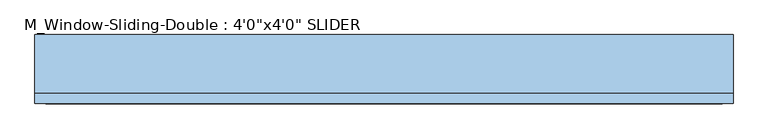
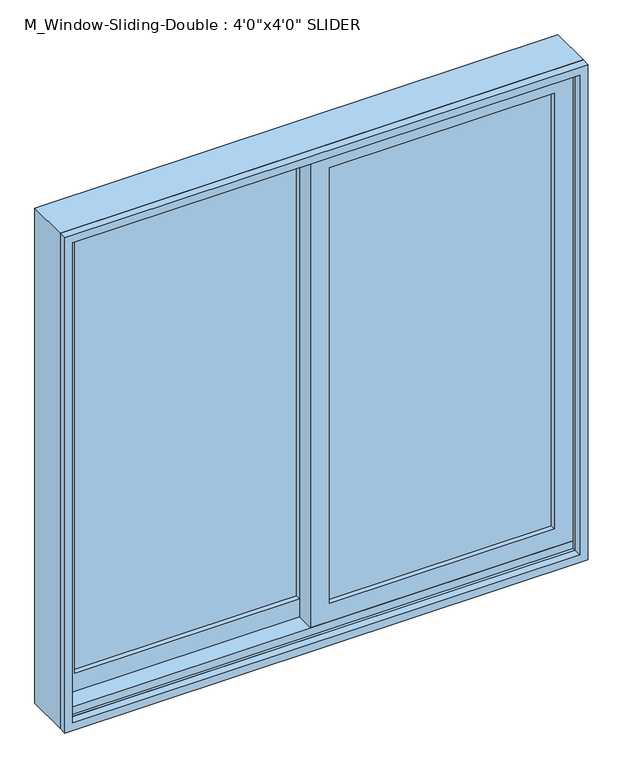
"""IFC4 building model written with IfcOpenShell, lengths in millimetres: window geometry."""

from ifc_helpers import new_model, si_unit, frame, origin, place, context, project, spatial, polyline, outline, extrude, faceted_brep, source, transform, mapped, element, save


def window_2d44019b(model_context):
    return source(origin(), model_context, "Body", "SolidModel", [
        faceted_brep([(-609.6, -35.56, 900.0), (-609.6, 66.04, 900.0), (609.6, 66.04, 900.0), (609.6, -35.56, 900.0), (-568.6778905, 66.04, 2078.2778905), (-568.6778905, 59.69, 2078.2778905), (-568.6778905, 59.69, 919.05), (-568.6778905, 66.04, 919.05), (568.6778905, 59.69, 2078.2778905), (568.6778905, 59.69, 919.05), (590.55, 59.69, 919.05), (590.55, 59.69, 2100.15), (-590.55, 59.69, 2100.15), (-590.55, 59.69, 919.05), (-590.55, -35.56, 2100.15), (-590.55, -35.56, 919.05), (-590.55, -29.21, 919.05), (-590.55, -29.21, 938.1), (-590.55, 15.24, 938.1), (-590.55, 15.24, 919.05), (609.6, -35.56, 2119.2), (-609.6, -35.56, 2119.2), (590.55, -35.56, 2100.15), (590.55, -35.56, 919.05), (-609.6, 66.04, 2119.2), (609.6, 66.04, 2119.2), (568.6778905, 66.04, 919.05), (568.6778905, 66.04, 2078.2778905), (590.55, 15.24, 919.05), (590.55, 15.24, 938.1), (590.55, -29.21, 938.1), (590.55, -29.21, 919.05)], [[[0, 1, 2, 3]], [[4, 5, 6, 7]], [[5, 8, 9, 10, 11, 12, 13, 6]], [[12, 14, 15, 16, 17, 18, 19, 13]], [[0, 3, 20, 21], [22, 23, 15, 14]], [[24, 1, 0, 21]], [[2, 1, 24, 25], [4, 7, 26, 27]], [[5, 4, 27, 8]], [[12, 11, 22, 14]], [[21, 20, 25, 24]], [[8, 27, 26, 9]], [[22, 11, 10, 28, 29, 30, 31, 23]], [[20, 3, 2, 25]], [[26, 7, 6, 13, 19, 28, 10, 9]], [[28, 19, 18, 29]], [[29, 18, 17, 30]], [[30, 17, 16, 31]], [[15, 23, 31, 16]]]),
        extrude(outline(polyline([(2119.2, -609.6), (900.0, -609.6), (900.0, 609.6), (2119.2, 609.6), (2119.2, -609.6)]), holes=[polyline([(2100.15, 590.55), (919.05, 590.55), (919.05, -590.55), (2100.15, -590.55), (2100.15, 590.55)])]), frame((0.0, -54.61, 0.0), z_axis=(0.0, 1.0, 0.0), x_axis=(0.0, 0.0, 1.0)), (0.0, 0.0, 1.0), 19.05),
        extrude(outline(polyline([(546.1, 2.54), (546.1, -3.81), (22.225, -3.81), (22.225, 2.54), (546.1, 2.54)])), frame((0.0, 0.0, 982.55), z_axis=(0.0, 0.0, 1.0), x_axis=(1.0, 0.0, 0.0)), (0.0, 0.0, 1.0), 1073.15),
        extrude(outline(polyline([(546.1, -10.16), (546.1, -16.51), (22.225, -16.51), (22.225, -10.16), (546.1, -10.16)])), frame((0.0, 0.0, 982.55), z_axis=(0.0, 0.0, 1.0), x_axis=(1.0, 0.0, 0.0)), (0.0, 0.0, 1.0), 1073.15),
        extrude(outline(polyline([(-22.225, 46.99), (-22.225, 40.64), (-546.1, 40.64), (-546.1, 46.99), (-22.225, 46.99)])), frame((0.0, 0.0, 982.55), z_axis=(0.0, 0.0, 1.0), x_axis=(1.0, 0.0, 0.0)), (0.0, 0.0, 1.0), 1073.15),
        extrude(outline(polyline([(-22.225, 34.29), (-22.225, 27.94), (-546.1, 27.94), (-546.1, 34.29), (-22.225, 34.29)])), frame((0.0, 0.0, 982.55), z_axis=(0.0, 0.0, 1.0), x_axis=(1.0, 0.0, 0.0)), (0.0, 0.0, 1.0), 1073.15),
        extrude(outline(polyline([(919.05, -590.55), (919.05, 22.225), (2100.15, 22.225), (2100.15, -590.55), (919.05, -590.55)]), holes=[polyline([(2055.7, -22.225), (982.55, -22.225), (982.55, -546.1), (2055.7, -546.1), (2055.7, -22.225)])]), frame((0.0, 15.24, 0.0), z_axis=(0.0, 1.0, 0.0), x_axis=(0.0, 0.0, 1.0)), (0.0, 0.0, 1.0), 44.45),
        extrude(outline(polyline([(938.1, 590.55), (2100.15, 590.55), (2100.15, -22.225), (938.1, -22.225), (938.1, 590.55)]), holes=[polyline([(982.55, 22.225), (2055.7, 22.225), (2055.7, 546.1), (982.55, 546.1), (982.55, 22.225)])]), frame((0.0, -29.21, 0.0), z_axis=(0.0, 1.0, 0.0), x_axis=(0.0, 0.0, 1.0)), (0.0, 0.0, 1.0), 44.45),
    ])


if __name__ == "__main__":
    model = new_model("IFC4")
    model_context = context("Model", 3, world=origin())
    ifc_project = project(units=[si_unit("LENGTHUNIT", "METRE", prefix="MILLI")], contexts=[model_context])
    site = spatial("IfcSite", under=ifc_project)
    building = spatial("IfcBuilding", under=site)
    placement = place(None, origin())
    window_shape = window_2d44019b(model_context)
    element("IfcWindow", 1, ObjectType="M_Window-Sliding-Double : 4'0\"x4'0\" SLIDER", at=placement, inside=building, context=model_context, shape_type="MappedRepresentation", body=[
        mapped(window_shape, transform((0.0, 0.0, 0.0), x_axis=(1.0, 0.0, 0.0), y_axis=(0.0, 1.0, 0.0), z_axis=(0.0, 0.0, 1.0))),
    ])
    save(model, "model.ifc")

# Revit data of these elements
# Type "M_Window-Sliding-Double : 4'0\"x4'0\" SLIDER"
#   Type Mark = "4"
#   Fire Rating = "0.5h"
#   Assembly Code = "B2020100"
#   Analytic Construction = "Double glazing - domestic"
#   Window Inset [instance default] = 0' - 0"
#   Wall Thickness [instance default] = 0' - 5.90551"
#   Visual Light Transmittance = 0.81
#   Thermal Resistance (R) = 1.8146 (h·ft²·°F)/BTU
#   Solar Heat Gain Coefficient = 0.76
#   Muntin Width = 1' - 8 5/8"
#   Muntin Height = 3' - 6 1/4"
#   Interior Wall Closure [instance default] = 0' - 2.65551"
#   Heat Transfer Coefficient (U) = 0.5511 BTU/(h·ft²·°F)
#   Frame Extension [instance default] = 0' - 0 1/4"
#   Exterior Wall Closure [instance default] = 0' - 1 1/4"
#   Rough Width = 4' - 0.59055"
#   Rough Height = 4' - 0.59055"
#   Height = 4' - 0"
#   Extension Jamb [instance default] = 0' - 2.65551"
#   Default Sill Height = 2' - 11.43307"
#   Width = 4' - 0"
#   Interior Trim Visibility [instance default] = yes
#   Indicator Visibility [instance default] = yes
#   Exterior Trim Visibility [instance default] = yes
#   Muntin Visibility = yes
#   Extension Jamb Visibility [instance default] = yes
#   Muntin Pattern = M_Muntin Pattern_2x2 : M_Muntin Pattern_2x2
#   Interior Trim Material = Wood - Stained
#   Interior Trim = M_Trim-Window-Interior-Flat : Picture Frame
#   Interior Frame Material = Wood - Stained
#   Glass Panel Material = Glass
#   Exterior Trim Material = Clad - White
#   Exterior Trim = M_Trim-Window-Exterior-Flat : with Sill
#   Exterior Frame Material = Clad - White
#   Wall Closure = (empty or 0)
# Element 1 (IfcWindow, "M_Window-Sliding-Double : 4'0\"x4'0\" SLIDER")
#   Wall Thickness = 0' - 4"
#   Extension Jamb = 0' - 0 3/4"
#   Materials on its faces: "Wood - Stained", "Glass", "Clad - White"
# Materials
#   "Wood - Stained": class "Wood", colour RGB 224 178 126, transparency 0, Cost = 0
#   "Glass": class "Glass", colour RGB 0 128 192, transparency 0.75, Description = "Soda Lime Glass", Cost = 0
#   "Clad - White": class "Wood", colour RGB 242 242 238, transparency 0, Cost = 0
